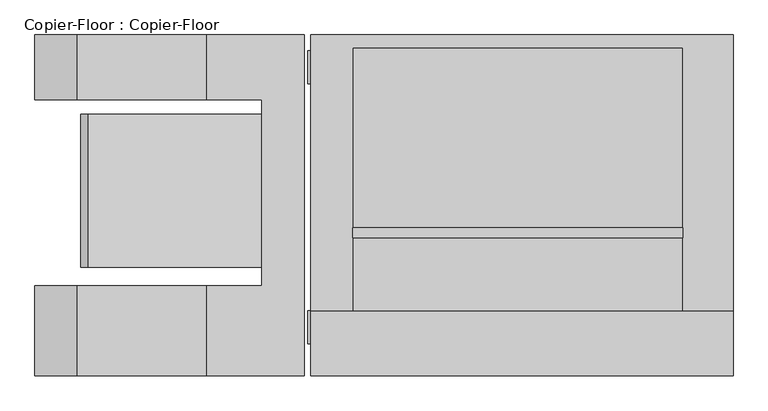
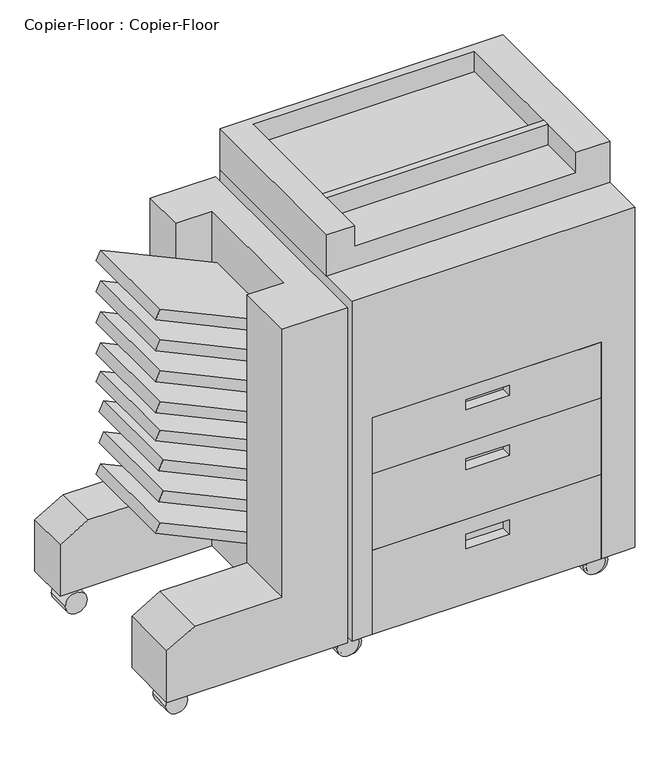
"""IFC4 building model written with IfcOpenShell, lengths in millimetres: proxy geometry, Copier-Floor : Copier-Floor."""

import ifcopenshell
import ifcopenshell.guid

model = None  # the IFC model being written
_history = None  # IfcOwnerHistory: only IFC2X3 demands one
_inside = {}  # id of a spatial element -> (the spatial element, [elements in it])
_under = {}  # id of a project, library or spatial element -> (it, [spatial elements below it])
_declared = {}  # id of a project -> (the project, [libraries it declares])
_typed = {}  # id of a type object -> (the type object, [elements of that type])
_made_of = {}  # id of a material, layer set ... -> (it, [elements and type objects made of it])


def new_model(schema):
    """Start an empty IFC model of exactly this schema.

    Asked for "IFC4X3", IfcOpenShell would pick the latest addendum, in which some entities
    have other attributes; the version numbers below select the first issue.
    IFC2X3 requires an IfcOwnerHistory on every rooted entity: one is made here for all.
    """
    global model, _history
    if schema == "IFC4X3":
        model = ifcopenshell.file(schema_version=(4, 3, 0, 0))
    else:
        model = ifcopenshell.file(schema=schema)
    _inside.clear()
    _under.clear()
    _declared.clear()
    _typed.clear()
    _made_of.clear()
    _history = None
    if model.schema == "IFC2X3":
        org = make("IfcOrganization", Name="unknown")
        user = make(
            "IfcPersonAndOrganization",
            ThePerson=make("IfcPerson", FamilyName="unknown"),
            TheOrganization=org,
        )
        app = make(
            "IfcApplication",
            ApplicationDeveloper=org,
            Version="unknown",
            ApplicationFullName="unknown",
            ApplicationIdentifier="unknown",
        )
        _history = make(
            "IfcOwnerHistory",
            OwningUser=user,
            OwningApplication=app,
            ChangeAction="ADDED",
            CreationDate=0,
        )
    return model


def make(cls, **values):
    """One entity of the class cls with the attributes given. An attribute that is None is left unset."""
    return model.create_entity(
        cls, **{name: value for name, value in values.items() if value is not None}
    )


def rooted(cls, **values):
    """An entity with a GlobalId (a new one), such as an element, a storey or a relation."""
    return make(cls, GlobalId=ifcopenshell.guid.new(), OwnerHistory=_history, **values)


def si_unit(unit_type, name, prefix=None):
    """IfcSIUnit, for example si_unit("LENGTHUNIT", "METRE", prefix="MILLI")."""
    return make("IfcSIUnit", UnitType=unit_type, Prefix=prefix, Name=name)


def assignment(units):
    """IfcUnitAssignment: the units of a project."""
    return None if units is None else make("IfcUnitAssignment", Units=units)


def point(xyz):
    """IfcCartesianPoint."""
    return None if xyz is None else make("IfcCartesianPoint", Coordinates=xyz)


def direction(xyz):
    """IfcDirection."""
    return None if xyz is None else make("IfcDirection", DirectionRatios=xyz)


def frame(location, z_axis=None, x_axis=None):
    """IfcAxis2Placement3D, a coordinate frame: its origin and axes. An axis left out is left unset."""
    return make(
        "IfcAxis2Placement3D",
        Location=point(location),
        Axis=direction(z_axis),
        RefDirection=direction(x_axis),
    )


def frame_2d(location, x_axis=None):
    """IfcAxis2Placement2D, a coordinate frame in the plane: its origin and x axis."""
    return make(
        "IfcAxis2Placement2D", Location=point(location), RefDirection=direction(x_axis)
    )


def origin():
    """The frame at (0, 0, 0) with its axes left unset."""
    return frame((0.0, 0.0, 0.0))


def place(relative_to, where):
    """IfcLocalPlacement: puts the frame where relative to a parent placement (None: the world)."""
    return make(
        "IfcLocalPlacement", PlacementRelTo=relative_to, RelativePlacement=where
    )


def context(
    kind, dimensions, precision=None, world=None, true_north=None, identifier=None
):
    """IfcGeometricRepresentationContext, for example the 3D "Model" context."""
    return make(
        "IfcGeometricRepresentationContext",
        ContextIdentifier=identifier,
        ContextType=kind,
        CoordinateSpaceDimension=dimensions,
        Precision=precision,
        WorldCoordinateSystem=world,
        TrueNorth=true_north,
    )


def project(units=None, contexts=None):
    """IfcProject with its units and contexts."""
    return rooted(
        "IfcProject",
        Name="project",
        RepresentationContexts=contexts,
        UnitsInContext=assignment(units),
    )


def spatial(cls, under=None, at=None, **own):
    """A site, building, storey or space (cls), placed at a placement, below another one or the project."""
    s = rooted(cls, ObjectPlacement=at, **own)
    if under is not None:
        _under.setdefault(under.id(), (under, []))[1].append(s)
    return s


def polyline(points):
    """IfcPolyline through the points."""
    return make("IfcPolyline", Points=[point(p) for p in points])


def circle_curve(where, radius):
    """IfcCircle in the frame where."""
    return make("IfcCircle", Position=where, Radius=radius)


def trimmed(basis, trim1, trim2, sense, master):
    """IfcTrimmedCurve: the piece of a basis curve between two trims."""
    return make(
        "IfcTrimmedCurve",
        BasisCurve=basis,
        Trim1=trim1,
        Trim2=trim2,
        SenseAgreement=sense,
        MasterRepresentation=master,
    )


def segment(curve, same_sense, transition):
    """IfcCompositeCurveSegment."""
    return make(
        "IfcCompositeCurveSegment",
        Transition=transition,
        SameSense=same_sense,
        ParentCurve=curve,
    )


def composite_curve(segments, self_intersect=None):
    """IfcCompositeCurve: segments joined end to end."""
    return make("IfcCompositeCurve", Segments=segments, SelfIntersect=self_intersect)


def outline(outer, holes=None, kind="AREA"):
    """IfcArbitraryClosedProfileDef: a profile drawn as a closed curve; with holes, ...WithVoids."""
    if holes is None:
        return make("IfcArbitraryClosedProfileDef", ProfileType=kind, OuterCurve=outer)
    return make(
        "IfcArbitraryProfileDefWithVoids",
        ProfileType=kind,
        OuterCurve=outer,
        InnerCurves=holes,
    )


def extrude(swept, where, along, depth):
    """IfcExtrudedAreaSolid: the profile swept, set in the frame where, extruded along a direction by depth."""
    return make(
        "IfcExtrudedAreaSolid",
        SweptArea=swept,
        Position=where,
        ExtrudedDirection=direction(along),
        Depth=depth,
    )


def faces_of(points, faces, orient=None, outer=None):
    """IfcFace entities. A face is a list of loops; a loop is a list of indices into points, from 0.

    orient and outer hold one flag for each loop. By default every Orientation is true, the
    first loop of a face is its IfcFaceOuterBound and the others are IfcFaceBound.
    """
    made = []
    for i, loops in enumerate(faces):
        bounds = []
        for j, loop in enumerate(loops):
            is_outer = j == 0 if outer is None else outer[i][j]
            bounds.append(
                make(
                    "IfcFaceOuterBound" if is_outer else "IfcFaceBound",
                    Bound=make("IfcPolyLoop", Polygon=[points[k] for k in loop]),
                    Orientation=True if orient is None else orient[i][j],
                )
            )
        made.append(make("IfcFace", Bounds=bounds))
    return made


def faceted_brep(points, faces, orient=None, outer=None, voids=None):
    """IfcFacetedBrep: a solid bounded by flat faces; with voids (closed shells), ...WithVoids."""
    shared = [point(p) for p in points]
    hull = make("IfcClosedShell", CfsFaces=faces_of(shared, faces, orient, outer))
    if voids is None:
        return make("IfcFacetedBrep", Outer=hull)
    return make(
        "IfcFacetedBrepWithVoids",
        Outer=hull,
        Voids=[
            make(cls, CfsFaces=faces_of(shared, fs, o, b)) for cls, fs, o, b in voids
        ],
    )


def shape(context_of_items, identifier, shape_type, items):
    """IfcShapeRepresentation: the items that make up one representation, for example the "Body"."""
    return make(
        "IfcShapeRepresentation",
        ContextOfItems=context_of_items,
        RepresentationIdentifier=identifier,
        RepresentationType=shape_type,
        Items=items,
    )


def source(mapping_origin, context_of_items, identifier, shape_type, items):
    """IfcRepresentationMap: a shape defined once, which mapped items show again and again."""
    return make(
        "IfcRepresentationMap",
        MappingOrigin=mapping_origin,
        MappedRepresentation=shape(context_of_items, identifier, shape_type, items),
    )


def transform(
    local_origin,
    x_axis=None,
    y_axis=None,
    z_axis=None,
    scale=None,
    scale2=None,
    scale3=None,
    uniform=True,
):
    """IfcCartesianTransformationOperator3D, or its non-uniform kind. x_axis, y_axis, z_axis: its Axis1, 2, 3."""
    if uniform:
        return make(
            "IfcCartesianTransformationOperator3D",
            Axis1=direction(x_axis),
            Axis2=direction(y_axis),
            LocalOrigin=point(local_origin),
            Scale=scale,
            Axis3=direction(z_axis),
        )
    return make(
        "IfcCartesianTransformationOperator3DnonUniform",
        Axis1=direction(x_axis),
        Axis2=direction(y_axis),
        LocalOrigin=point(local_origin),
        Scale=scale,
        Axis3=direction(z_axis),
        Scale2=scale2,
        Scale3=scale3,
    )


def mapped(mapping_source, mapping_target):
    """IfcMappedItem: shows the shape of a source again, moved by a transform."""
    return make(
        "IfcMappedItem", MappingSource=mapping_source, MappingTarget=mapping_target
    )


def made_of(thing, what):
    """Note that an element or type object is made of a material, layer set ...; save() writes the relation."""
    if what is not None:
        _made_of.setdefault(what.id(), (what, []))[1].append(thing)
    return thing


def element(
    cls,
    number,
    at=None,
    inside=None,
    cuts=None,
    type_object=None,
    material=None,
    context=None,
    identifier="Body",
    shape_type=None,
    held_by="IfcProductDefinitionShape",
    body=None,
    shapes=None,
    **own,
):
    """One element of the class cls, such as IfcWall. Its Tag is "e" and its number.

    at: its placement. inside: the storey or other place that contains it. cuts: it is an
    opening in that element (IfcRelVoidsElement). A single representation is given by context,
    identifier, shape_type and body (its items); several are given by shapes. held_by: the class
    of the entity that holds the representations. save() writes the other relations.
    """
    e = rooted(cls, Tag="e%d" % number, ObjectPlacement=at, **own)
    if body is not None:
        shapes = [shape(context, identifier, shape_type, body)]
    if shapes is not None:
        e.Representation = make(held_by, Representations=shapes)
    if inside is not None:
        _inside.setdefault(inside.id(), (inside, []))[1].append(e)
    if cuts is not None:
        rooted(
            "IfcRelVoidsElement", RelatingBuildingElement=cuts, RelatedOpeningElement=e
        )
    if type_object is not None:
        _typed.setdefault(type_object.id(), (type_object, []))[1].append(e)
    return made_of(e, material)


def aggregate(whole, parts):
    """IfcRelAggregates: a whole, such as a stair, and the parts it consists of."""
    return rooted("IfcRelAggregates", RelatingObject=whole, RelatedObjects=parts)


def save(model, path):
    """Write the relations noted so far, then the file.

    IfcRelAggregates (storeys below a building ...), IfcRelContainedInSpatialStructure (elements
    in a storey), IfcRelDefinesByType, IfcRelAssociatesMaterial and IfcRelDeclares: one each for
    every whole, place, type object, material and project.
    """
    for whole, parts in _under.values():
        aggregate(whole, parts)
    for where, things in _inside.values():
        rooted(
            "IfcRelContainedInSpatialStructure",
            RelatedElements=things,
            RelatingStructure=where,
        )
    for kind, things in _typed.values():
        rooted("IfcRelDefinesByType", RelatedObjects=things, RelatingType=kind)
    for what, things in _made_of.values():
        rooted("IfcRelAssociatesMaterial", RelatedObjects=things, RelatingMaterial=what)
    for by, libraries in _declared.values():
        rooted("IfcRelDeclares", RelatingContext=by, RelatedDefinitions=libraries)
    model.write(path)


def copier_floor_copier_floor_a40bf9c1(model_context):
    return source(origin(), model_context, "Body", "SolidModel", [
        extrude(outline(polyline([(387.7567294, -681.6535349), (364.7365116, -692.3880388), (232.9041289, -409.6725817), (260.929928, -409.6725817), (387.7567294, -681.6535349)])), frame((0.0, -72.1685532, 0.0), z_axis=(0.0, 1.0, 0.0), x_axis=(0.0, 0.0, 1.0)), (0.0, 0.0, 1.0), 239.8222339),
        extrude(outline(polyline([(463.6667654, -675.0122673), (440.6465476, -685.7467712), (311.9110388, -409.6725817), (339.9368379, -409.6725817), (463.6667654, -675.0122673)])), frame((0.0, -72.1685532, 0.0), z_axis=(0.0, 1.0, 0.0), x_axis=(0.0, 0.0, 1.0)), (0.0, 0.0, 1.0), 239.8222339),
        extrude(outline(polyline([(539.8667654, -675.0122673), (516.8465476, -685.7467712), (388.1110388, -409.6725817), (416.1368379, -409.6725817), (539.8667654, -675.0122673)])), frame((0.0, -72.1685532, 0.0), z_axis=(0.0, 1.0, 0.0), x_axis=(0.0, 0.0, 1.0)), (0.0, 0.0, 1.0), 239.8222339),
        extrude(outline(polyline([(914.2268014, -681.6535349), (891.2065836, -692.3880388), (759.3742009, -409.6725817), (787.4, -409.6725817), (914.2268014, -681.6535349)])), frame((0.0, -72.1685532, 0.0), z_axis=(0.0, 1.0, 0.0), x_axis=(0.0, 0.0, 1.0)), (0.0, 0.0, 1.0), 239.8222339),
        extrude(outline(polyline([(838.0268014, -681.6535349), (815.0065836, -692.3880388), (683.1742009, -409.6725817), (711.2, -409.6725817), (838.0268014, -681.6535349)])), frame((0.0, -72.1685532, 0.0), z_axis=(0.0, 1.0, 0.0), x_axis=(0.0, 0.0, 1.0)), (0.0, 0.0, 1.0), 239.8222339),
        extrude(outline(polyline([(615.7768014, -681.6535349), (592.7565836, -692.3880388), (460.9242009, -409.6725817), (488.95, -409.6725817), (615.7768014, -681.6535349)])), frame((0.0, -72.1685532, 0.0), z_axis=(0.0, 1.0, 0.0), x_axis=(0.0, 0.0, 1.0)), (0.0, 0.0, 1.0), 239.8222339),
        extrude(outline(polyline([(685.6268014, -681.6535349), (662.6065836, -692.3880388), (530.7742009, -409.6725817), (558.8, -409.6725817), (685.6268014, -681.6535349)])), frame((0.0, -72.1685532, 0.0), z_axis=(0.0, 1.0, 0.0), x_axis=(0.0, 0.0, 1.0)), (0.0, 0.0, 1.0), 239.8222339),
        extrude(outline(polyline([(761.8268014, -681.6535349), (738.8065836, -692.3880388), (606.9742009, -409.6725817), (635.0, -409.6725817), (761.8268014, -681.6535349)])), frame((0.0, -72.1685532, 0.0), z_axis=(0.0, 1.0, 0.0), x_axis=(0.0, 0.0, 1.0)), (0.0, 0.0, 1.0), 239.8222339),
        extrude(outline(composite_curve([segment(trimmed(circle_curve(frame_2d((26.0668925, -711.8709821)), 25.4), [point((26.0668925, -737.2709821))], [point((26.0668925, -686.4709821))], False, "CARTESIAN"), True, "CONTINUOUS"), segment(trimmed(circle_curve(frame_2d((26.0668925, -711.8709821)), 25.4), [point((26.0668925, -686.4709821))], [point((26.0668925, -737.2709821))], False, "CARTESIAN"), True, "CONTINUOUS")], self_intersect=False)), frame((0.0, 215.1689468, 0.0), z_axis=(0.0, 1.0, 0.0), x_axis=(0.0, 0.0, 1.0)), (0.0, 0.0, 1.0), 55.9418879),
        extrude(outline(composite_curve([segment(trimmed(circle_curve(frame_2d((26.0668925, -711.8709821)), 25.4), [point((26.0668925, -737.2709821))], [point((26.0668925, -686.4709821))], False, "CARTESIAN"), True, "CONTINUOUS"), segment(trimmed(circle_curve(frame_2d((26.0668925, -711.8709821)), 25.4), [point((26.0668925, -686.4709821))], [point((26.0668925, -737.2709821))], False, "CARTESIAN"), True, "CONTINUOUS")], self_intersect=False)), frame((0.0, -191.2310532, 0.0), z_axis=(0.0, 1.0, 0.0), x_axis=(0.0, 0.0, 1.0)), (0.0, 0.0, 1.0), 51.3258053),
        faceted_brep([(-764.1654582, -242.0310532, 76.2), (-342.5743224, -242.0310532, 76.2), (-342.5743224, -242.0310532, 901.7), (-494.9743224, -242.0310532, 901.7), (-494.9743224, -242.0310532, 241.3), (-698.1743224, -242.0310532, 241.3), (-764.1654582, -242.0310532, 203.2), (-764.1654582, 291.3689468, 76.2), (-764.1654582, 291.3689468, 203.2), (-698.1743224, 291.3689468, 241.3), (-494.9743224, 291.3689468, 241.3), (-494.9743224, 291.3689468, 901.7), (-342.5743224, 291.3689468, 901.7), (-342.5743224, 291.3689468, 76.2), (-764.1654582, -100.8888364, 76.2), (-409.6725817, -100.8888364, 76.2), (-409.6725817, 189.7689468, 76.2), (-764.1654582, 189.7689468, 76.2), (-494.9743224, 189.7689468, 901.7), (-409.6725817, 189.7689468, 901.7), (-409.6725817, -100.8888364, 901.7), (-494.9743224, -100.8888364, 901.7), (-494.9743224, -100.8888364, 241.3), (-494.9743224, 189.7689468, 241.3), (-698.1743224, -100.8888364, 241.3), (-698.1743224, 189.7689468, 241.3), (-764.1654582, -100.8888364, 203.2), (-764.1654582, 189.7689468, 203.2)], [[[0, 1, 2, 3, 4, 5, 6]], [[7, 8, 9, 10, 11, 12, 13]], [[1, 0, 14, 15, 16, 17, 7, 13]], [[2, 1, 13, 12]], [[3, 2, 12, 11, 18, 19, 20, 21]], [[4, 3, 21, 22]], [[11, 10, 23, 18]], [[5, 4, 22, 24]], [[10, 9, 25, 23]], [[6, 5, 24, 26]], [[9, 8, 27, 25]], [[0, 6, 26, 14]], [[8, 7, 17, 27]], [[16, 19, 18, 23, 25, 27, 17]], [[20, 15, 14, 26, 24, 22, 21]], [[19, 16, 15, 20]]]),
        extrude(outline(composite_curve([segment(trimmed(circle_curve(frame_2d((27.9129458, -312.2555429)), 25.4), [point((27.9129458, -337.6555429))], [point((27.9129458, -286.8555429))], False, "CARTESIAN"), True, "CONTINUOUS"), segment(trimmed(circle_curve(frame_2d((27.9129458, -312.2555429)), 25.4), [point((27.9129458, -286.8555429))], [point((27.9129458, -337.6555429))], False, "CARTESIAN"), True, "CONTINUOUS")], self_intersect=False)), frame((0.0, 215.1689468, 0.0), z_axis=(0.0, 1.0, 0.0), x_axis=(0.0, 0.0, 1.0)), (0.0, 0.0, 1.0), 51.3258053),
        extrude(outline(composite_curve([segment(trimmed(circle_curve(frame_2d((27.9129458, 262.7398948)), 25.4), [point((27.9129458, 237.3398948))], [point((27.9129458, 288.1398948))], False, "CARTESIAN"), True, "CONTINUOUS"), segment(trimmed(circle_curve(frame_2d((27.9129458, 262.7398948)), 25.4), [point((27.9129458, 288.1398948))], [point((27.9129458, 237.3398948))], False, "CARTESIAN"), True, "CONTINUOUS")], self_intersect=False)), frame((0.0, 215.1689468, 0.0), z_axis=(0.0, 1.0, 0.0), x_axis=(0.0, 0.0, 1.0)), (0.0, 0.0, 1.0), 51.3258053),
        extrude(outline(composite_curve([segment(trimmed(circle_curve(frame_2d((27.9129458, -312.2555429)), 25.4), [point((27.9129458, -337.6555429))], [point((27.9129458, -286.8555429))], False, "CARTESIAN"), True, "CONTINUOUS"), segment(trimmed(circle_curve(frame_2d((27.9129458, -312.2555429)), 25.4), [point((27.9129458, -286.8555429))], [point((27.9129458, -337.6555429))], False, "CARTESIAN"), True, "CONTINUOUS")], self_intersect=False)), frame((0.0, -191.2310532, 0.0), z_axis=(0.0, 1.0, 0.0), x_axis=(0.0, 0.0, 1.0)), (0.0, 0.0, 1.0), 51.3258053),
        extrude(outline(composite_curve([segment(trimmed(circle_curve(frame_2d((27.9129458, 262.7398948)), 25.4), [point((27.9129458, 237.3398948))], [point((27.9129458, 288.1398948))], False, "CARTESIAN"), True, "CONTINUOUS"), segment(trimmed(circle_curve(frame_2d((27.9129458, 262.7398948)), 25.4), [point((27.9129458, 288.1398948))], [point((27.9129458, 237.3398948))], False, "CARTESIAN"), True, "CONTINUOUS")], self_intersect=False)), frame((0.0, -191.2310532, 0.0), z_axis=(0.0, 1.0, 0.0), x_axis=(0.0, 0.0, 1.0)), (0.0, 0.0, 1.0), 51.3258053),
        extrude(outline(composite_curve([segment(trimmed(circle_curve(frame_2d((27.9129458, -306.6302391)), 25.4), [point((27.9129458, -332.0302391))], [point((27.9129458, -281.2302391))], False, "CARTESIAN"), True, "CONTINUOUS"), segment(trimmed(circle_curve(frame_2d((27.9129458, -306.6302391)), 25.4), [point((27.9129458, -281.2302391))], [point((27.9129458, -332.0302391))], False, "CARTESIAN"), True, "CONTINUOUS")], self_intersect=False)), frame((0.0, -191.2310532, 0.0), z_axis=(0.0, 1.0, 0.0), x_axis=(0.0, 0.0, 1.0)), (0.0, 0.0, 1.0), 51.3258053),
        extrude(outline(composite_curve([segment(trimmed(circle_curve(frame_2d((27.9129458, 268.3651986)), 25.4), [point((27.9129458, 242.9651986))], [point((27.9129458, 293.7651986))], False, "CARTESIAN"), True, "CONTINUOUS"), segment(trimmed(circle_curve(frame_2d((27.9129458, 268.3651986)), 25.4), [point((27.9129458, 293.7651986))], [point((27.9129458, 242.9651986))], False, "CARTESIAN"), True, "CONTINUOUS")], self_intersect=False)), frame((0.0, -191.2310532, 0.0), z_axis=(0.0, 1.0, 0.0), x_axis=(0.0, 0.0, 1.0)), (0.0, 0.0, 1.0), 51.3258053),
        extrude(outline(polyline([(249.314028, -26.1310532), (-267.2959958, -26.1310532), (-267.2959958, -10.0577181), (249.314028, -10.0577181), (249.314028, -26.1310532)])), frame((0.0, 0.0, 965.2), z_axis=(0.0, 0.0, 1.0), x_axis=(1.0, 0.0, 0.0)), (0.0, 0.0, 1.0), 50.8),
        faceted_brep([(249.314028, -242.0310532, 472.3553727), (249.314028, -242.0310532, 609.6), (-284.085972, -242.0310532, 609.6), (-284.085972, -242.0310532, 472.3553727), (-66.7741493, -242.0310532, 578.8591447), (34.8258507, -242.0310532, 578.8591447), (34.8258507, -242.0310532, 553.4591447), (-66.7741493, -242.0310532, 553.4591447), (249.314028, -191.2310532, 472.3553727), (-284.085972, -191.2310532, 472.3553727), (-284.085972, -191.2310532, 609.6), (249.314028, -191.2310532, 609.6), (34.8258507, -216.6310532, 578.8591447), (-66.7741493, -216.6310532, 578.8591447), (-66.7741493, -216.6310532, 553.4591447), (34.8258507, -216.6310532, 553.4591447)], [[[0, 1, 2, 3], [4, 5, 6, 7]], [[8, 9, 10, 11]], [[1, 0, 8, 11]], [[2, 1, 11, 10]], [[3, 2, 10, 9]], [[0, 3, 9, 8]], [[12, 13, 14, 15]], [[13, 12, 5, 4]], [[14, 13, 4, 7]], [[15, 14, 7, 6]], [[12, 15, 6, 5]]]),
        faceted_brep([(249.314028, -242.0310532, 283.8723489), (249.314028, -242.0310532, 472.3553727), (-284.085972, -242.0310532, 472.3553727), (-284.085972, -242.0310532, 283.8723489), (-66.7741493, -242.0310532, 432.3774172), (34.8258507, -242.0310532, 432.3774172), (34.8258507, -242.0310532, 406.4), (-66.7741493, -242.0310532, 406.4), (249.314028, -191.2310532, 283.8723489), (-284.085972, -191.2310532, 283.8723489), (-284.085972, -191.2310532, 472.3553727), (249.314028, -191.2310532, 472.3553727), (34.8258507, -216.6310532, 432.3774172), (-66.7741493, -216.6310532, 432.3774172), (-66.7741493, -216.6310532, 406.4), (34.8258507, -216.6310532, 406.4)], [[[0, 1, 2, 3], [4, 5, 6, 7]], [[8, 9, 10, 11]], [[1, 0, 8, 11]], [[2, 1, 11, 10]], [[3, 2, 10, 9]], [[0, 3, 9, 8]], [[12, 13, 14, 15]], [[13, 12, 5, 4]], [[14, 13, 4, 7]], [[15, 14, 7, 6]], [[12, 15, 6, 5]]]),
        faceted_brep([(249.314028, -242.0310532, 76.2), (249.314028, -242.0310532, 283.8723489), (-284.085972, -242.0310532, 283.8723489), (-284.085972, -242.0310532, 76.2), (-66.7741493, -242.0310532, 246.5423898), (34.8258507, -242.0310532, 246.5423898), (34.8258507, -242.0310532, 211.1096445), (-66.7741493, -242.0310532, 211.1096445), (249.314028, -191.2310532, 76.2), (-284.085972, -191.2310532, 76.2), (-284.085972, -191.2310532, 283.8723489), (249.314028, -191.2310532, 283.8723489), (34.8258507, -216.6310532, 246.5423898), (-66.7741493, -216.6310532, 246.5423898), (-66.7741493, -216.6310532, 211.1096445), (34.8258507, -216.6310532, 211.1096445)], [[[0, 1, 2, 3], [4, 5, 6, 7]], [[8, 9, 10, 11]], [[1, 0, 8, 11]], [[2, 1, 11, 10]], [[3, 2, 10, 9]], [[0, 3, 9, 8]], [[12, 13, 14, 15]], [[13, 12, 5, 4]], [[14, 13, 4, 7]], [[15, 14, 7, 6]], [[12, 15, 6, 5]]]),
        faceted_brep([(328.0345418, 291.3689468, 1016.0), (-332.3654582, 291.3689468, 1016.0), (-332.3654582, -139.9052479, 1016.0), (-267.2959958, -139.9052479, 1016.0), (-267.2959958, 271.1108348, 1016.0), (249.314028, 271.1108348, 1016.0), (249.314028, -139.9052479, 1016.0), (328.0345418, -139.9052479, 1016.0), (328.0345418, 291.3689468, 914.4), (328.0345418, -139.9052479, 914.4), (-332.3654582, -139.9052479, 914.4), (-332.3654582, 291.3689468, 914.4), (249.314028, -139.9052479, 965.2), (-267.2959958, -139.9052479, 965.2), (249.314028, 271.1108348, 965.2), (-267.2959958, 271.1108348, 965.2)], [[[0, 1, 2, 3, 4, 5, 6, 7]], [[8, 9, 10, 11]], [[1, 0, 8, 11]], [[2, 1, 11, 10]], [[10, 9, 7, 6, 12, 13, 3, 2]], [[0, 7, 9, 8]], [[14, 15, 13, 12]], [[15, 14, 5, 4]], [[13, 15, 4, 3]], [[14, 12, 6, 5]]]),
        faceted_brep([(328.0345418, 291.3689468, 914.4), (-332.3654582, 291.3689468, 914.4), (-332.3654582, -242.0310532, 914.4), (328.0345418, -242.0310532, 914.4), (328.0345418, 291.3689468, 76.2), (328.0345418, -242.0310532, 76.2), (249.314028, -242.0310532, 76.2), (249.314028, -191.2310532, 76.2), (-284.085972, -191.2310532, 76.2), (-284.085972, -242.0310532, 76.2), (-332.3654582, -242.0310532, 76.2), (-332.3654582, 291.3689468, 76.2), (-284.085972, -242.0310532, 609.6), (249.314028, -242.0310532, 609.6), (-284.085972, -191.2310532, 609.6), (249.314028, -191.2310532, 609.6)], [[[0, 1, 2, 3]], [[4, 5, 6, 7, 8, 9, 10, 11]], [[1, 0, 4, 11]], [[2, 1, 11, 10]], [[3, 2, 10, 9, 12, 13, 6, 5]], [[0, 3, 5, 4]], [[14, 8, 7, 15]], [[8, 14, 12, 9]], [[15, 7, 6, 13]], [[14, 15, 13, 12]]]),
    ])


if __name__ == "__main__":
    model = new_model("IFC4")
    model_context = context("Model", 3, world=origin())
    ifc_project = project(units=[si_unit("LENGTHUNIT", "METRE", prefix="MILLI")], contexts=[model_context])
    site = spatial("IfcSite", under=ifc_project)
    building = spatial("IfcBuilding", under=site)
    placement = place(None, origin())
    copier_floor_copier_floor_shape = copier_floor_copier_floor_a40bf9c1(model_context)
    element("IfcBuildingElementProxy", 1, Name="Copier-Floor : Copier-Floor", ObjectType="Copier-Floor : Copier-Floor", at=placement, inside=building, context=model_context, shape_type="MappedRepresentation", body=[
        mapped(copier_floor_copier_floor_shape, transform((0.0, 0.0, 0.0), x_axis=(1.0, 0.0, 0.0), y_axis=(0.0, 1.0, 0.0), z_axis=(0.0, 0.0, 1.0))),
    ])
    save(model, "model.ifc")

# Revit data of these elements
# Type "Copier-Floor : Copier-Floor"
#   Assembly Code = "E1010800"
#   Default Elevation = 0
# Element 1 (IfcBuildingElementProxy, "Copier-Floor : Copier-Floor")
#   Materials on its faces: "Plastic - White", "Plastic - Gray,Dark"
# Materials
#   "Plastic - White": class "Unassigned", colour RGB 249 232 210, transparency 0
#   "Plastic - Gray,Dark": class "Unassigned", colour RGB 134 134 134, transparency 0
